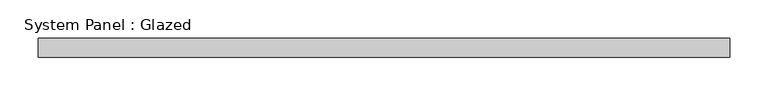
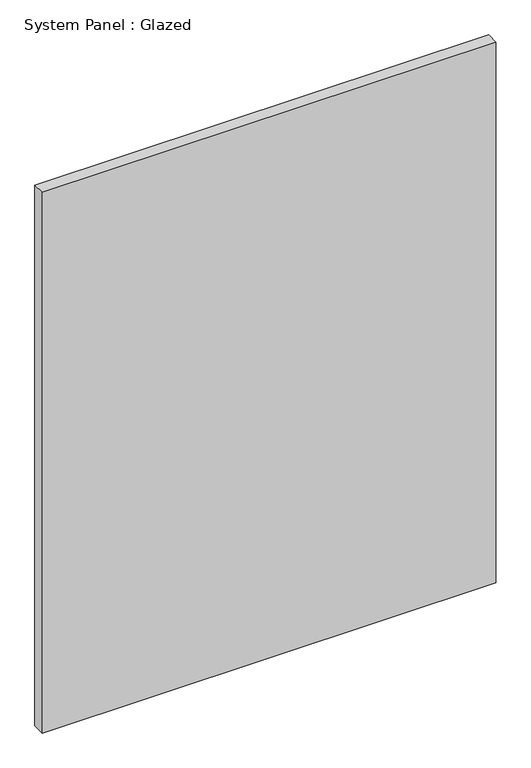
"""IFC4 building model written with IfcOpenShell, lengths in millimetres: plate geometry, System Panel : Glazed."""

from ifc_helpers import new_model, si_unit, origin, origin_with_axes, place, context, project, spatial, polyline, outline, extrude, source, transform, mapped, element, save


def system_panel_glazed_ace91e9e(model_context):
    return source(origin(), model_context, "Body", "SweptSolid", [
        extrude(outline(polyline([(453.5714285, -12.7), (-453.5714285, -12.7), (-453.5714285, 12.7), (453.5714285, 12.7), (453.5714285, -12.7)])), origin_with_axes(), (0.0, 0.0, 1.0), 1143.0),
    ])


if __name__ == "__main__":
    model = new_model("IFC4")
    model_context = context("Model", 3, world=origin())
    ifc_project = project(units=[si_unit("LENGTHUNIT", "METRE", prefix="MILLI")], contexts=[model_context])
    site = spatial("IfcSite", under=ifc_project)
    building = spatial("IfcBuilding", under=site)
    placement = place(None, origin())
    system_panel_glazed_shape = system_panel_glazed_ace91e9e(model_context)
    element("IfcPlate", 1, ObjectType="System Panel : Glazed", at=placement, inside=building, context=model_context, shape_type="MappedRepresentation", body=[
        mapped(system_panel_glazed_shape, transform((0.0, 0.0, 0.0), x_axis=(1.0, 0.0, 0.0), y_axis=(0.0, 1.0, 0.0), z_axis=(0.0, 0.0, 1.0))),
    ])
    save(model, "model.ifc")

# Revit data of these elements
# Element 1 (IfcPlate, "System Panel : Glazed")
#   Materials on its faces: "Glass"
# Materials
#   "Glass": class "Glass", colour RGB 218 227 224, transparency 0.85, Description = "Soda Lime Glass", Cost = 0
